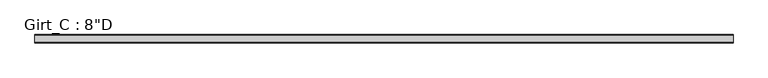
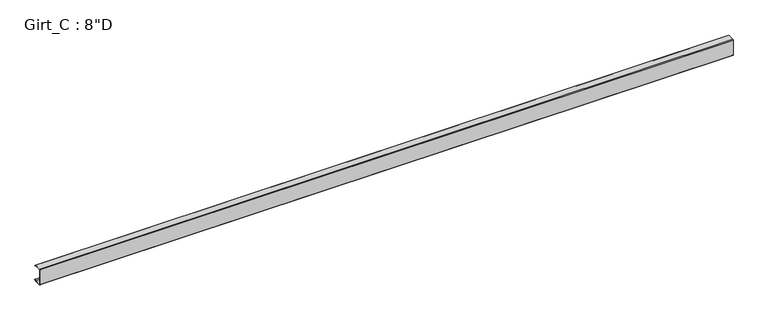
"""IFC4 building model written with IfcOpenShell, lengths in millimetres: beam geometry."""

import ifcopenshell
import ifcopenshell.guid

model = None  # the IFC model being written
_history = None  # IfcOwnerHistory: only IFC2X3 demands one
_inside = {}  # id of a spatial element -> (the spatial element, [elements in it])
_under = {}  # id of a project, library or spatial element -> (it, [spatial elements below it])
_declared = {}  # id of a project -> (the project, [libraries it declares])
_typed = {}  # id of a type object -> (the type object, [elements of that type])
_made_of = {}  # id of a material, layer set ... -> (it, [elements and type objects made of it])


def new_model(schema):
    """Start an empty IFC model of exactly this schema.

    Asked for "IFC4X3", IfcOpenShell would pick the latest addendum, in which some entities
    have other attributes; the version numbers below select the first issue.
    IFC2X3 requires an IfcOwnerHistory on every rooted entity: one is made here for all.
    """
    global model, _history
    if schema == "IFC4X3":
        model = ifcopenshell.file(schema_version=(4, 3, 0, 0))
    else:
        model = ifcopenshell.file(schema=schema)
    _inside.clear()
    _under.clear()
    _declared.clear()
    _typed.clear()
    _made_of.clear()
    _history = None
    if model.schema == "IFC2X3":
        org = make("IfcOrganization", Name="unknown")
        user = make(
            "IfcPersonAndOrganization",
            ThePerson=make("IfcPerson", FamilyName="unknown"),
            TheOrganization=org,
        )
        app = make(
            "IfcApplication",
            ApplicationDeveloper=org,
            Version="unknown",
            ApplicationFullName="unknown",
            ApplicationIdentifier="unknown",
        )
        _history = make(
            "IfcOwnerHistory",
            OwningUser=user,
            OwningApplication=app,
            ChangeAction="ADDED",
            CreationDate=0,
        )
    return model


def make(cls, **values):
    """One entity of the class cls with the attributes given. An attribute that is None is left unset."""
    return model.create_entity(
        cls, **{name: value for name, value in values.items() if value is not None}
    )


def rooted(cls, **values):
    """An entity with a GlobalId (a new one), such as an element, a storey or a relation."""
    return make(cls, GlobalId=ifcopenshell.guid.new(), OwnerHistory=_history, **values)


def si_unit(unit_type, name, prefix=None):
    """IfcSIUnit, for example si_unit("LENGTHUNIT", "METRE", prefix="MILLI")."""
    return make("IfcSIUnit", UnitType=unit_type, Prefix=prefix, Name=name)


def assignment(units):
    """IfcUnitAssignment: the units of a project."""
    return None if units is None else make("IfcUnitAssignment", Units=units)


def point(xyz):
    """IfcCartesianPoint."""
    return None if xyz is None else make("IfcCartesianPoint", Coordinates=xyz)


def direction(xyz):
    """IfcDirection."""
    return None if xyz is None else make("IfcDirection", DirectionRatios=xyz)


def frame(location, z_axis=None, x_axis=None):
    """IfcAxis2Placement3D, a coordinate frame: its origin and axes. An axis left out is left unset."""
    return make(
        "IfcAxis2Placement3D",
        Location=point(location),
        Axis=direction(z_axis),
        RefDirection=direction(x_axis),
    )


def frame_2d(location, x_axis=None):
    """IfcAxis2Placement2D, a coordinate frame in the plane: its origin and x axis."""
    return make(
        "IfcAxis2Placement2D", Location=point(location), RefDirection=direction(x_axis)
    )


def origin():
    """The frame at (0, 0, 0) with its axes left unset."""
    return frame((0.0, 0.0, 0.0))


def place(relative_to, where):
    """IfcLocalPlacement: puts the frame where relative to a parent placement (None: the world)."""
    return make(
        "IfcLocalPlacement", PlacementRelTo=relative_to, RelativePlacement=where
    )


def context(
    kind, dimensions, precision=None, world=None, true_north=None, identifier=None
):
    """IfcGeometricRepresentationContext, for example the 3D "Model" context."""
    return make(
        "IfcGeometricRepresentationContext",
        ContextIdentifier=identifier,
        ContextType=kind,
        CoordinateSpaceDimension=dimensions,
        Precision=precision,
        WorldCoordinateSystem=world,
        TrueNorth=true_north,
    )


def project(units=None, contexts=None):
    """IfcProject with its units and contexts."""
    return rooted(
        "IfcProject",
        Name="project",
        RepresentationContexts=contexts,
        UnitsInContext=assignment(units),
    )


def spatial(cls, under=None, at=None, **own):
    """A site, building, storey or space (cls), placed at a placement, below another one or the project."""
    s = rooted(cls, ObjectPlacement=at, **own)
    if under is not None:
        _under.setdefault(under.id(), (under, []))[1].append(s)
    return s


def polyline(points):
    """IfcPolyline through the points."""
    return make("IfcPolyline", Points=[point(p) for p in points])


def circle_curve(where, radius):
    """IfcCircle in the frame where."""
    return make("IfcCircle", Position=where, Radius=radius)


def trimmed(basis, trim1, trim2, sense, master):
    """IfcTrimmedCurve: the piece of a basis curve between two trims."""
    return make(
        "IfcTrimmedCurve",
        BasisCurve=basis,
        Trim1=trim1,
        Trim2=trim2,
        SenseAgreement=sense,
        MasterRepresentation=master,
    )


def segment(curve, same_sense, transition):
    """IfcCompositeCurveSegment."""
    return make(
        "IfcCompositeCurveSegment",
        Transition=transition,
        SameSense=same_sense,
        ParentCurve=curve,
    )


def composite_curve(segments, self_intersect=None):
    """IfcCompositeCurve: segments joined end to end."""
    return make("IfcCompositeCurve", Segments=segments, SelfIntersect=self_intersect)


def outline(outer, holes=None, kind="AREA"):
    """IfcArbitraryClosedProfileDef: a profile drawn as a closed curve; with holes, ...WithVoids."""
    if holes is None:
        return make("IfcArbitraryClosedProfileDef", ProfileType=kind, OuterCurve=outer)
    return make(
        "IfcArbitraryProfileDefWithVoids",
        ProfileType=kind,
        OuterCurve=outer,
        InnerCurves=holes,
    )


def extrude(swept, where, along, depth):
    """IfcExtrudedAreaSolid: the profile swept, set in the frame where, extruded along a direction by depth."""
    return make(
        "IfcExtrudedAreaSolid",
        SweptArea=swept,
        Position=where,
        ExtrudedDirection=direction(along),
        Depth=depth,
    )


def shape(context_of_items, identifier, shape_type, items):
    """IfcShapeRepresentation: the items that make up one representation, for example the "Body"."""
    return make(
        "IfcShapeRepresentation",
        ContextOfItems=context_of_items,
        RepresentationIdentifier=identifier,
        RepresentationType=shape_type,
        Items=items,
    )


def source(mapping_origin, context_of_items, identifier, shape_type, items):
    """IfcRepresentationMap: a shape defined once, which mapped items show again and again."""
    return make(
        "IfcRepresentationMap",
        MappingOrigin=mapping_origin,
        MappedRepresentation=shape(context_of_items, identifier, shape_type, items),
    )


def transform(
    local_origin,
    x_axis=None,
    y_axis=None,
    z_axis=None,
    scale=None,
    scale2=None,
    scale3=None,
    uniform=True,
):
    """IfcCartesianTransformationOperator3D, or its non-uniform kind. x_axis, y_axis, z_axis: its Axis1, 2, 3."""
    if uniform:
        return make(
            "IfcCartesianTransformationOperator3D",
            Axis1=direction(x_axis),
            Axis2=direction(y_axis),
            LocalOrigin=point(local_origin),
            Scale=scale,
            Axis3=direction(z_axis),
        )
    return make(
        "IfcCartesianTransformationOperator3DnonUniform",
        Axis1=direction(x_axis),
        Axis2=direction(y_axis),
        LocalOrigin=point(local_origin),
        Scale=scale,
        Axis3=direction(z_axis),
        Scale2=scale2,
        Scale3=scale3,
    )


def mapped(mapping_source, mapping_target):
    """IfcMappedItem: shows the shape of a source again, moved by a transform."""
    return make(
        "IfcMappedItem", MappingSource=mapping_source, MappingTarget=mapping_target
    )


def made_of(thing, what):
    """Note that an element or type object is made of a material, layer set ...; save() writes the relation."""
    if what is not None:
        _made_of.setdefault(what.id(), (what, []))[1].append(thing)
    return thing


def element(
    cls,
    number,
    at=None,
    inside=None,
    cuts=None,
    type_object=None,
    material=None,
    context=None,
    identifier="Body",
    shape_type=None,
    held_by="IfcProductDefinitionShape",
    body=None,
    shapes=None,
    **own,
):
    """One element of the class cls, such as IfcWall. Its Tag is "e" and its number.

    at: its placement. inside: the storey or other place that contains it. cuts: it is an
    opening in that element (IfcRelVoidsElement). A single representation is given by context,
    identifier, shape_type and body (its items); several are given by shapes. held_by: the class
    of the entity that holds the representations. save() writes the other relations.
    """
    e = rooted(cls, Tag="e%d" % number, ObjectPlacement=at, **own)
    if body is not None:
        shapes = [shape(context, identifier, shape_type, body)]
    if shapes is not None:
        e.Representation = make(held_by, Representations=shapes)
    if inside is not None:
        _inside.setdefault(inside.id(), (inside, []))[1].append(e)
    if cuts is not None:
        rooted(
            "IfcRelVoidsElement", RelatingBuildingElement=cuts, RelatedOpeningElement=e
        )
    if type_object is not None:
        _typed.setdefault(type_object.id(), (type_object, []))[1].append(e)
    return made_of(e, material)


def aggregate(whole, parts):
    """IfcRelAggregates: a whole, such as a stair, and the parts it consists of."""
    return rooted("IfcRelAggregates", RelatingObject=whole, RelatedObjects=parts)


def save(model, path):
    """Write the relations noted so far, then the file.

    IfcRelAggregates (storeys below a building ...), IfcRelContainedInSpatialStructure (elements
    in a storey), IfcRelDefinesByType, IfcRelAssociatesMaterial and IfcRelDeclares: one each for
    every whole, place, type object, material and project.
    """
    for whole, parts in _under.values():
        aggregate(whole, parts)
    for where, things in _inside.values():
        rooted(
            "IfcRelContainedInSpatialStructure",
            RelatedElements=things,
            RelatingStructure=where,
        )
    for kind, things in _typed.values():
        rooted("IfcRelDefinesByType", RelatedObjects=things, RelatingType=kind)
    for what, things in _made_of.values():
        rooted("IfcRelAssociatesMaterial", RelatedObjects=things, RelatingMaterial=what)
    for by, libraries in _declared.values():
        rooted("IfcRelDeclares", RelatingContext=by, RelatedDefinitions=libraries)
    model.write(path)


def beam_3fe9278c(model_context):
    return source(origin(), model_context, "Body", "SweptSolid", [
        extrude(outline(composite_curve([segment(polyline([(87.5109375, 101.6), (99.7560415, 87.0068534), (97.6278742, 85.221109), (86.2154765, 98.821875), (3.3005807, 98.821875)]), True, "CONTINUOUS"), segment(trimmed(circle_curve(frame_2d((3.3741066, 96.8381931)), 1.9850441), [point((3.3005807, 98.821875))], [point((1.3890625, 96.8381931))], True, "CARTESIAN"), True, "CONTINUOUS"), segment(polyline([(1.3890625, 96.8381931), (1.3890625, -96.8389339)]), True, "CONTINUOUS"), segment(trimmed(circle_curve(frame_2d((3.3748024, -96.8389339)), 1.9857399), [point((1.3890625, -96.8389339))], [point((3.2694106, -98.821875))], True, "CARTESIAN"), True, "CONTINUOUS"), segment(polyline([(3.2694106, -98.821875), (86.2154765, -98.821875), (97.6510975, -85.1934327), (99.7792647, -86.979177), (87.5109375, -101.6), (3.3734375, -101.6)]), True, "CONTINUOUS"), segment(trimmed(circle_curve(frame_2d((3.3734375, -96.8375)), 4.7625), [point((3.3734375, -101.6))], [point((-1.3890625, -96.8375))], False, "CARTESIAN"), True, "CONTINUOUS"), segment(polyline([(-1.3890625, -96.8375), (-1.3890625, 96.8375)]), True, "CONTINUOUS"), segment(trimmed(circle_curve(frame_2d((3.3734375, 96.8375)), 4.7625), [point((-1.3890625, 96.8375))], [point((3.3734375, 101.6))], False, "CARTESIAN"), True, "CONTINUOUS"), segment(polyline([(3.3734375, 101.6), (87.5109375, 101.6)]), True, "CONTINUOUS")], self_intersect=False)), frame((-4206.5723786, 0.0, 0.0), z_axis=(1.0, 0.0, 0.0), x_axis=(0.0, 1.0, 0.0)), (0.0, 0.0, 1.0), 8444.8947573),
    ])


if __name__ == "__main__":
    model = new_model("IFC4")
    model_context = context("Model", 3, world=origin())
    ifc_project = project(units=[si_unit("LENGTHUNIT", "METRE", prefix="MILLI")], contexts=[model_context])
    site = spatial("IfcSite", under=ifc_project)
    building = spatial("IfcBuilding", under=site)
    placement = place(None, origin())
    beam_shape = beam_3fe9278c(model_context)
    element("IfcBeam", 1, ObjectType="Girt_C : 8\"D", at=placement, inside=building, context=model_context, shape_type="MappedRepresentation", body=[
        mapped(beam_shape, transform((0.0, 0.0, 0.0), x_axis=(1.0, 0.0, 0.0), y_axis=(0.0, 1.0, 0.0), z_axis=(0.0, 0.0, 1.0))),
    ])
    save(model, "model.ifc")

# Revit data of these elements
# Type "Girt_C : 8\"D"
#   half leg = 0' - 1 3/4"
#   Web_Thickness = 0' - 0 7/64"
#   Length [instance default] = 10' - 0"
#   Leg_1 = 0' - 3 1/2"
#   Height = 0' - 8"
#   Structural Material [instance default] = none
# Element 1 (IfcBeam, "Girt_C : 8\"D")
#   Structural Material = GALVANIZED 'CEE' SECTION (8.0x3.5C - SEE STRUCT. DWGS)
#   Materials on its faces: "GALVANIZED 'CEE' SECTION (8.0x3.5C - SEE STRUCT. DWGS)"
# Materials
#   "GALVANIZED 'CEE' SECTION (8.0x3.5C - SEE STRUCT. DWGS)": class "Metal", colour RGB 137 146 153, transparency 0, Description = "Steel, mill finish", Cost = 0
